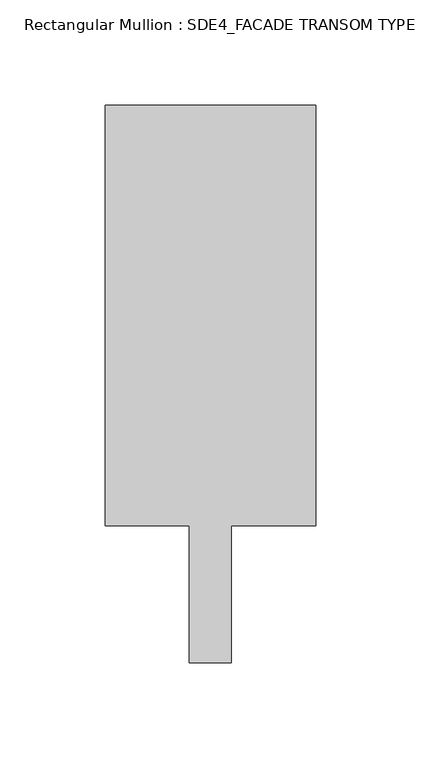
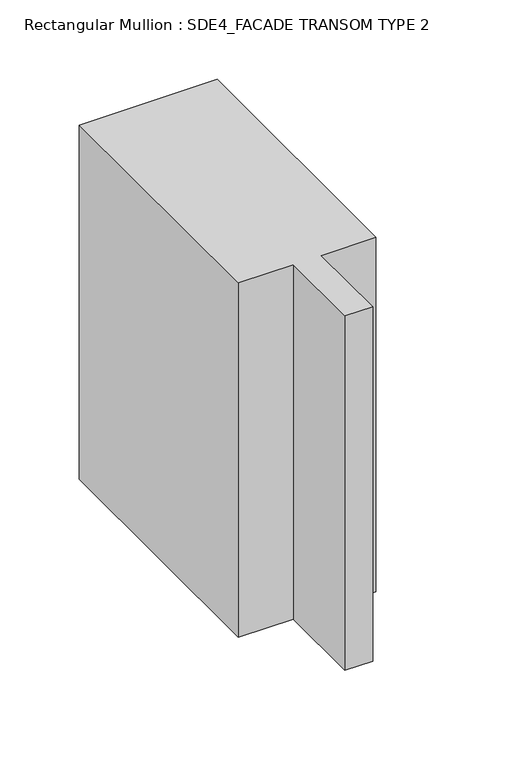
"""IFC4 building model written with IfcOpenShell, lengths in millimetres: member geometry, Rectangular Mullion : SDE4_FACADE TRANSOM TYPE 2."""

from ifc_helpers import new_model, si_unit, frame, origin, place, context, project, spatial, polyline, outline, extrude, source, transform, mapped, element, save


def rectangular_mullion_sde4_facade_transom_type_2_67608d63(model_context):
    return source(origin(), model_context, "Body", "SweptSolid", [
        extrude(outline(polyline([(50.0, 132.5), (50.0, -67.5), (10.0, -67.5), (10.0, -132.5), (-10.0, -132.5), (-10.0, -67.5), (-50.0, -67.5), (-50.0, 132.5), (50.0, 132.5)])), frame((0.0, 0.0, -272.3185505), z_axis=(0.0, 0.0, 1.0), x_axis=(1.0, 0.0, 0.0)), (0.0, 0.0, 1.0), 272.3185505),
    ])


if __name__ == "__main__":
    model = new_model("IFC4")
    model_context = context("Model", 3, world=origin())
    ifc_project = project(units=[si_unit("LENGTHUNIT", "METRE", prefix="MILLI")], contexts=[model_context])
    site = spatial("IfcSite", under=ifc_project)
    building = spatial("IfcBuilding", under=site)
    placement = place(None, origin())
    rectangular_mullion_sde4_facade_transom_type_2_shape = rectangular_mullion_sde4_facade_transom_type_2_67608d63(model_context)
    element("IfcMember", 1, ObjectType="Rectangular Mullion : SDE4_FACADE TRANSOM TYPE 2", at=placement, inside=building, context=model_context, shape_type="MappedRepresentation", body=[
        mapped(rectangular_mullion_sde4_facade_transom_type_2_shape, transform((0.0, 0.0, 0.0), x_axis=(1.0, 0.0, 0.0), y_axis=(0.0, 1.0, 0.0), z_axis=(0.0, 0.0, 1.0))),
    ])
    save(model, "model.ifc")

# Revit data of these elements
# Type "Rectangular Mullion : SDE4_FACADE TRANSOM TYPE 2"
#   built-in parameter 1007322 = 0.869423 (stored number, unit not read)
#   built-in parameter 1007321 = 0.164042 (stored number, unit not read)
#   built-in parameter 1007320 = 0.164042 (stored number, unit not read)
